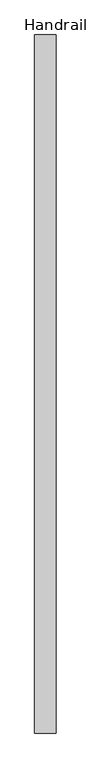
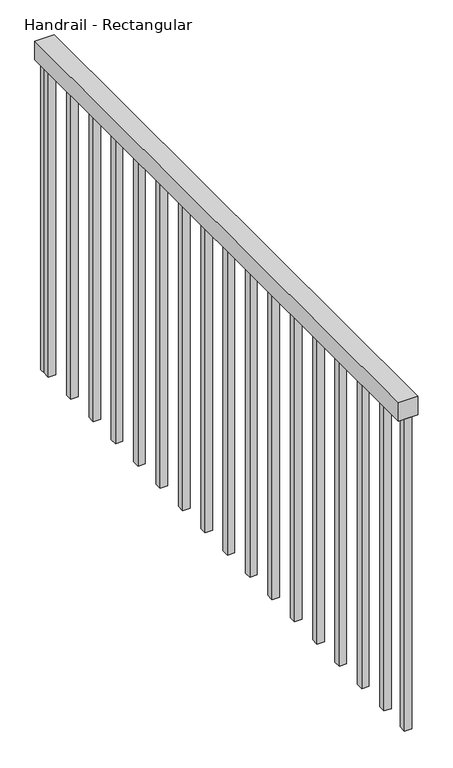
"""IFC4 building model written with IfcOpenShell, lengths in millimetres: railing geometry, Handrail - Rectangular."""

from ifc_helpers import new_model, si_unit, frame, origin, place, context, project, spatial, polyline, outline, extrude, source, transform, mapped, element, save


def handrail_rectangular_9e89d571(model_context):
    return source(origin(), model_context, "Body", "SweptSolid", [
        extrude(outline(polyline([(-12364.4211091, 6945.8507146), (-12415.2211091, 6945.8507146), (-12415.2211091, 8595.8507146), (-12364.4211091, 8595.8507146), (-12364.4211091, 6945.8507146)])), frame((0.0, 0.0, 6654.4), z_axis=(0.0, 0.0, 1.0), x_axis=(1.0, 0.0, 0.0)), (0.0, 0.0, 1.0), 50.8),
        extrude(outline(polyline([(-12380.2961091, 8561.9257146), (-12399.3461091, 8561.9257146), (-12399.3461091, 8580.9757146), (-12380.2961091, 8580.9757146), (-12380.2961091, 8561.9257146)])), frame((0.0, 0.0, 5790.8), z_axis=(0.0, 0.0, 1.0), x_axis=(1.0, 0.0, 0.0)), (0.0, 0.0, 1.0), 863.6),
        extrude(outline(polyline([(-12380.2961091, 8460.3257146), (-12399.3461091, 8460.3257146), (-12399.3461091, 8479.3757146), (-12380.2961091, 8479.3757146), (-12380.2961091, 8460.3257146)])), frame((0.0, 0.0, 5790.8), z_axis=(0.0, 0.0, 1.0), x_axis=(1.0, 0.0, 0.0)), (0.0, 0.0, 1.0), 863.6),
        extrude(outline(polyline([(-12380.2961091, 8358.7257146), (-12399.3461091, 8358.7257146), (-12399.3461091, 8377.7757146), (-12380.2961091, 8377.7757146), (-12380.2961091, 8358.7257146)])), frame((0.0, 0.0, 5790.8), z_axis=(0.0, 0.0, 1.0), x_axis=(1.0, 0.0, 0.0)), (0.0, 0.0, 1.0), 863.6),
        extrude(outline(polyline([(-12380.2961091, 8257.1257146), (-12399.3461091, 8257.1257146), (-12399.3461091, 8276.1757146), (-12380.2961091, 8276.1757146), (-12380.2961091, 8257.1257146)])), frame((0.0, 0.0, 5790.8), z_axis=(0.0, 0.0, 1.0), x_axis=(1.0, 0.0, 0.0)), (0.0, 0.0, 1.0), 863.6),
        extrude(outline(polyline([(-12380.2961091, 8155.5257146), (-12399.3461091, 8155.5257146), (-12399.3461091, 8174.5757146), (-12380.2961091, 8174.5757146), (-12380.2961091, 8155.5257146)])), frame((0.0, 0.0, 5790.8), z_axis=(0.0, 0.0, 1.0), x_axis=(1.0, 0.0, 0.0)), (0.0, 0.0, 1.0), 863.6),
        extrude(outline(polyline([(-12380.2961091, 8053.9257146), (-12399.3461091, 8053.9257146), (-12399.3461091, 8072.9757146), (-12380.2961091, 8072.9757146), (-12380.2961091, 8053.9257146)])), frame((0.0, 0.0, 5790.8), z_axis=(0.0, 0.0, 1.0), x_axis=(1.0, 0.0, 0.0)), (0.0, 0.0, 1.0), 863.6),
        extrude(outline(polyline([(-12380.2961091, 7952.3257146), (-12399.3461091, 7952.3257146), (-12399.3461091, 7971.3757146), (-12380.2961091, 7971.3757146), (-12380.2961091, 7952.3257146)])), frame((0.0, 0.0, 5790.8), z_axis=(0.0, 0.0, 1.0), x_axis=(1.0, 0.0, 0.0)), (0.0, 0.0, 1.0), 863.6),
        extrude(outline(polyline([(-12380.2961091, 7850.7257146), (-12399.3461091, 7850.7257146), (-12399.3461091, 7869.7757146), (-12380.2961091, 7869.7757146), (-12380.2961091, 7850.7257146)])), frame((0.0, 0.0, 5790.8), z_axis=(0.0, 0.0, 1.0), x_axis=(1.0, 0.0, 0.0)), (0.0, 0.0, 1.0), 863.6),
        extrude(outline(polyline([(-12380.2961091, 7749.1257146), (-12399.3461091, 7749.1257146), (-12399.3461091, 7768.1757146), (-12380.2961091, 7768.1757146), (-12380.2961091, 7749.1257146)])), frame((0.0, 0.0, 5790.8), z_axis=(0.0, 0.0, 1.0), x_axis=(1.0, 0.0, 0.0)), (0.0, 0.0, 1.0), 863.6),
        extrude(outline(polyline([(-12380.2961091, 7647.5257146), (-12399.3461091, 7647.5257146), (-12399.3461091, 7666.5757146), (-12380.2961091, 7666.5757146), (-12380.2961091, 7647.5257146)])), frame((0.0, 0.0, 5790.8), z_axis=(0.0, 0.0, 1.0), x_axis=(1.0, 0.0, 0.0)), (0.0, 0.0, 1.0), 863.6),
        extrude(outline(polyline([(-12380.2961091, 7545.9257146), (-12399.3461091, 7545.9257146), (-12399.3461091, 7564.9757146), (-12380.2961091, 7564.9757146), (-12380.2961091, 7545.9257146)])), frame((0.0, 0.0, 5790.8), z_axis=(0.0, 0.0, 1.0), x_axis=(1.0, 0.0, 0.0)), (0.0, 0.0, 1.0), 863.6),
        extrude(outline(polyline([(-12380.2961091, 7444.3257146), (-12399.3461091, 7444.3257146), (-12399.3461091, 7463.3757146), (-12380.2961091, 7463.3757146), (-12380.2961091, 7444.3257146)])), frame((0.0, 0.0, 5790.8), z_axis=(0.0, 0.0, 1.0), x_axis=(1.0, 0.0, 0.0)), (0.0, 0.0, 1.0), 863.6),
        extrude(outline(polyline([(-12380.2961091, 7342.7257146), (-12399.3461091, 7342.7257146), (-12399.3461091, 7361.7757146), (-12380.2961091, 7361.7757146), (-12380.2961091, 7342.7257146)])), frame((0.0, 0.0, 5790.8), z_axis=(0.0, 0.0, 1.0), x_axis=(1.0, 0.0, 0.0)), (0.0, 0.0, 1.0), 863.6),
        extrude(outline(polyline([(-12380.2961091, 7241.1257146), (-12399.3461091, 7241.1257146), (-12399.3461091, 7260.1757146), (-12380.2961091, 7260.1757146), (-12380.2961091, 7241.1257146)])), frame((0.0, 0.0, 5790.8), z_axis=(0.0, 0.0, 1.0), x_axis=(1.0, 0.0, 0.0)), (0.0, 0.0, 1.0), 863.6),
        extrude(outline(polyline([(-12380.2961091, 7139.5257146), (-12399.3461091, 7139.5257146), (-12399.3461091, 7158.5757146), (-12380.2961091, 7158.5757146), (-12380.2961091, 7139.5257146)])), frame((0.0, 0.0, 5790.8), z_axis=(0.0, 0.0, 1.0), x_axis=(1.0, 0.0, 0.0)), (0.0, 0.0, 1.0), 863.6),
        extrude(outline(polyline([(-12380.2961091, 7037.9257146), (-12399.3461091, 7037.9257146), (-12399.3461091, 7056.9757146), (-12380.2961091, 7056.9757146), (-12380.2961091, 7037.9257146)])), frame((0.0, 0.0, 5790.8), z_axis=(0.0, 0.0, 1.0), x_axis=(1.0, 0.0, 0.0)), (0.0, 0.0, 1.0), 863.6),
        extrude(outline(polyline([(-12380.2961091, 8576.8007146), (-12399.3461091, 8576.8007146), (-12399.3461091, 8595.8507146), (-12380.2961091, 8595.8507146), (-12380.2961091, 8576.8007146)])), frame((0.0, 0.0, 5790.8), z_axis=(0.0, 0.0, 1.0), x_axis=(1.0, 0.0, 0.0)), (0.0, 0.0, 1.0), 863.6),
        extrude(outline(polyline([(-12380.2961091, 6945.8507146), (-12399.3461091, 6945.8507146), (-12399.3461091, 6964.9007146), (-12380.2961091, 6964.9007146), (-12380.2961091, 6945.8507146)])), frame((0.0, 0.0, 5790.8), z_axis=(0.0, 0.0, 1.0), x_axis=(1.0, 0.0, 0.0)), (0.0, 0.0, 1.0), 863.6),
    ])


if __name__ == "__main__":
    model = new_model("IFC4")
    model_context = context("Model", 3, world=origin())
    ifc_project = project(units=[si_unit("LENGTHUNIT", "METRE", prefix="MILLI")], contexts=[model_context])
    site = spatial("IfcSite", under=ifc_project)
    building = spatial("IfcBuilding", under=site)
    placement = place(None, origin())
    handrail_rectangular_shape = handrail_rectangular_9e89d571(model_context)
    element("IfcRailing", 1, ObjectType="Handrail - Rectangular", at=placement, inside=building, context=model_context, shape_type="MappedRepresentation", body=[
        mapped(handrail_rectangular_shape, transform((0.0, 0.0, 0.0), x_axis=(1.0, 0.0, 0.0), y_axis=(0.0, 1.0, 0.0), z_axis=(0.0, 0.0, 1.0))),
    ])
    save(model, "model.ifc")
